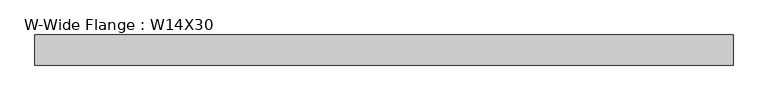
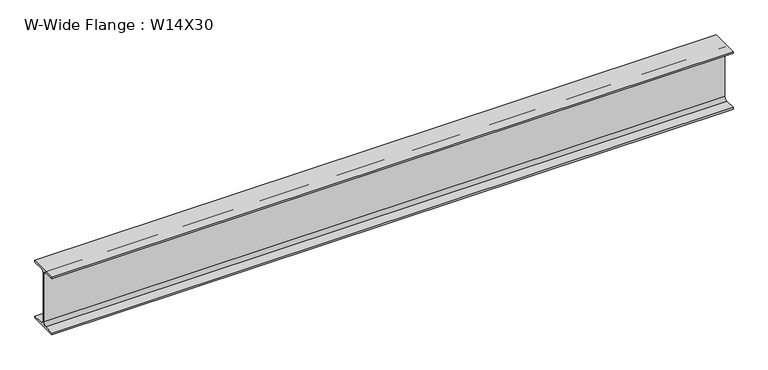
"""IFC4 building model written with IfcOpenShell, lengths in millimetres: beam geometry, W-Wide Flange : W14X30."""

from ifc_helpers import new_model, si_unit, point, frame, frame_2d, origin, place, context, project, spatial, polyline, circle_curve, trimmed, segment, composite_curve, outline, extrude, source, transform, mapped, element, save


def w_wide_flange_w14x30_17857959(model_context):
    return source(origin(), model_context, "Body", "SweptSolid", [
        extrude(outline(composite_curve([segment(polyline([(85.4769531, -165.9433594), (85.4769531, -175.7660156), (-85.4769531, -175.7660156), (-85.4769531, -165.9433594), (-22.1753906, -165.9433594)]), True, "CONTINUOUS"), segment(trimmed(circle_curve(frame_2d((-22.1753906, -147.1910156)), 18.7523438), [point((-22.1753906, -165.9433594))], [point((-3.4230469, -147.1910156))], True, "CARTESIAN"), True, "CONTINUOUS"), segment(polyline([(-3.4230469, -147.1910156), (-3.4230469, 147.1910156)]), True, "CONTINUOUS"), segment(trimmed(circle_curve(frame_2d((-22.1753906, 147.1910156)), 18.7523438), [point((-3.4230469, 147.1910156))], [point((-22.1753906, 165.9433594))], True, "CARTESIAN"), True, "CONTINUOUS"), segment(polyline([(-22.1753906, 165.9433594), (-85.4769531, 165.9433594), (-85.4769531, 175.7660156), (85.4769531, 175.7660156), (85.4769531, 165.9433594), (22.1753906, 165.9433594)]), True, "CONTINUOUS"), segment(trimmed(circle_curve(frame_2d((22.1753906, 147.1910156)), 18.7523438), [point((22.1753906, 165.9433594))], [point((3.4230469, 147.1910156))], True, "CARTESIAN"), True, "CONTINUOUS"), segment(polyline([(3.4230469, 147.1910156), (3.4230469, -147.1910156)]), True, "CONTINUOUS"), segment(trimmed(circle_curve(frame_2d((22.1753906, -147.1910156)), 18.7523438), [point((3.4230469, -147.1910156))], [point((22.1753906, -165.9433594))], True, "CARTESIAN"), True, "CONTINUOUS"), segment(polyline([(22.1753906, -165.9433594), (85.4769531, -165.9433594)]), True, "CONTINUOUS")], self_intersect=False)), frame((-1963.4835, 0.0, 0.0), z_axis=(1.0, 0.0, 0.0), x_axis=(0.0, 1.0, 0.0)), (0.0, 0.0, 1.0), 3956.0440469),
    ])


if __name__ == "__main__":
    model = new_model("IFC4")
    model_context = context("Model", 3, world=origin())
    ifc_project = project(units=[si_unit("LENGTHUNIT", "METRE", prefix="MILLI")], contexts=[model_context])
    site = spatial("IfcSite", under=ifc_project)
    building = spatial("IfcBuilding", under=site)
    placement = place(None, origin())
    w_wide_flange_w14x30_shape = w_wide_flange_w14x30_17857959(model_context)
    element("IfcBeam", 1, ObjectType="W-Wide Flange : W14X30", at=placement, inside=building, context=model_context, shape_type="MappedRepresentation", body=[
        mapped(w_wide_flange_w14x30_shape, transform((0.0, 0.0, 0.0), x_axis=(1.0, 0.0, 0.0), y_axis=(0.0, 1.0, 0.0), z_axis=(0.0, 0.0, 1.0))),
    ])
    save(model, "model.ifc")

# Revit data of these elements
# Type "W-Wide Flange : W14X30"
#   Assembly Code = "B10"
#   W = 30
#   Length [instance default] = 1524 mm
#   bf = 170.954 mm
#   d = 351.532 mm
#   k = 28.575 mm
#   k2 = 18.752 mm
#   tf = 9.823 mm
#   tw = 6.846 mm
#   A = 0.00557418 m²
#   Structural Material [instance default] = Steel ASTM A992
# Element 1 (IfcBeam, "W-Wide Flange : W14X30")
#   Structural Material = Aluminum, Anodized Red
#   Materials on its faces: "Aluminum, Anodized Red"
# Materials
#   "Steel ASTM A992": class "Metal", colour RGB 128 0 0, transparency 0, Description = "Structural steel 50ksi", Cost = 0
#   "Aluminum, Anodized Red": class "Metal", colour RGB 120 120 120, transparency 0, Description = "Anodized aluminum, red", Cost = 0
